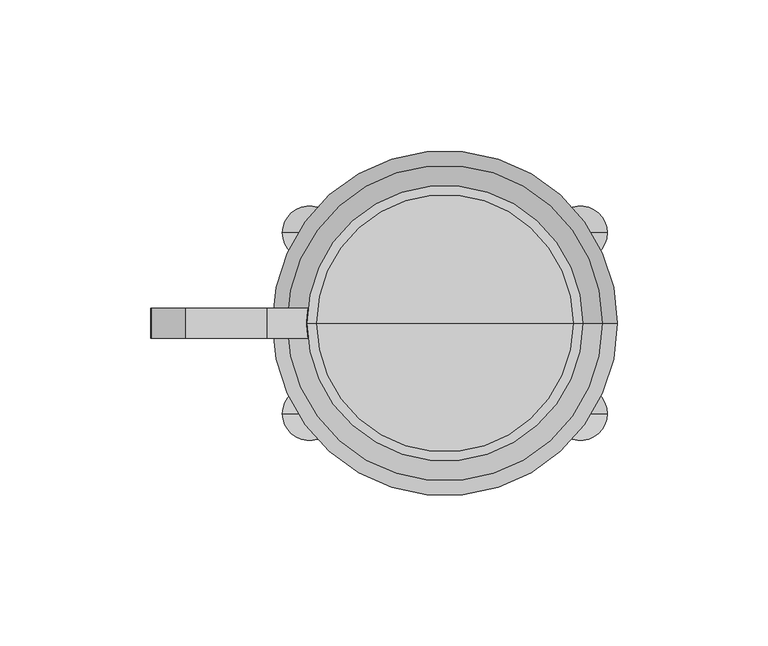
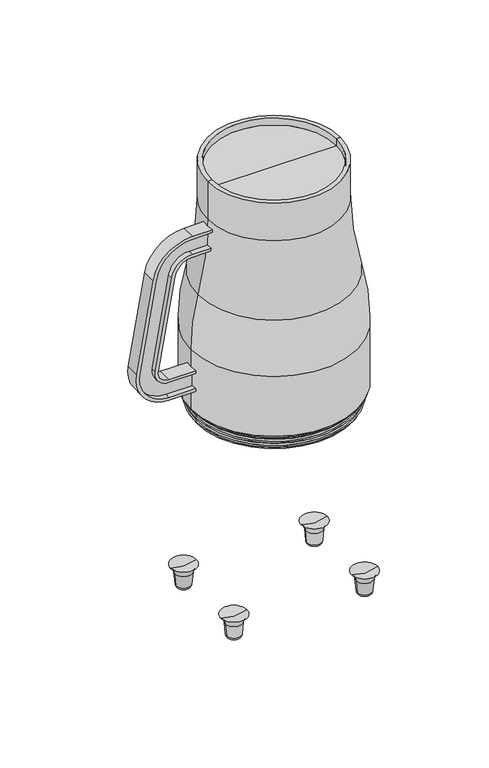
"""IFC4 building model written with IfcOpenShell, lengths in millimetres: proxy geometry, Smoothie_Maker_ : Smoothie_Maker_."""

from ifc_helpers import new_model, si_unit, point, frame, origin, place, context, project, spatial, polyline, circle_curve, ellipse_curve, trimmed, source, transform, mapped, element, save
from ifc_brep_helpers import plane_surface, cylinder_surface, revolved_surface, advanced_brep


def generic_models_ff15e8bf(model_context):
    return source(origin(), model_context, "Body", "AdvancedBrep", [
        advanced_brep(
        [(-43.932782, 5.0, 280.5), (-43.932782, -5.0, 280.5), (-43.932782, -5.0, 278.5), (-43.932782, -1.0, 278.5), (-43.932782, -1.0, 267.5), (-43.932782, -5.0, 267.5), (-43.932782, -5.0, 265.5), (-43.932782, 5.0, 265.5), (-43.932782, 5.0, 267.5), (-43.932782, 1.0, 267.5), (-43.932782, 1.0, 278.5), (-43.932782, 5.0, 278.5), (-58.932782, 5.0, 280.5), (-58.932782, -5.0, 280.5), (-86.0149953, -5.0, 257.7753249), (-97.361463, -5.0, 193.4263087), (-75.2032886, -5.0, 167.0192247), (-55.2032886, -5.0, 167.0192247), (-55.2032886, -5.0, 169.0192247), (-75.2032886, -5.0, 169.0192247), (-95.3918475, -5.0, 193.0790123), (-84.0453798, -5.0, 257.4280285), (-58.932782, -5.0, 278.5), (-58.932782, -1.0, 278.5), (-84.0453798, -1.0, 257.4280285), (-95.3918475, -1.0, 193.0790123), (-75.2032886, -1.0, 169.0192247), (-55.2032886, -1.0, 169.0192247), (-55.2032886, -1.0, 180.0192247), (-75.2032886, -1.0, 180.0192247), (-84.5589622, -1.0, 191.1688824), (-73.2124945, -1.0, 255.5178986), (-58.932782, -1.0, 267.5), (-58.932782, -5.0, 267.5), (-73.2124945, -5.0, 255.5178986), (-84.5589622, -5.0, 191.1688824), (-75.2032886, -5.0, 180.0192247), (-55.2032886, -5.0, 180.0192247), (-55.2032886, -5.0, 182.0192247), (-75.2032886, -5.0, 182.0192247), (-82.5893467, -5.0, 190.821586), (-71.242879, -5.0, 255.1706022), (-58.932782, -5.0, 265.5), (-58.932782, 5.0, 265.5), (-71.242879, 5.0, 255.1706022), (-82.5893467, 5.0, 190.821586), (-75.2032886, 5.0, 182.0192247), (-55.2032886, 5.0, 182.0192247), (-55.2032886, 5.0, 180.0192247), (-75.2032886, 5.0, 180.0192247), (-84.5589622, 5.0, 191.1688824), (-73.2124945, 5.0, 255.5178986), (-58.932782, 5.0, 267.5), (-58.932782, 1.0, 267.5), (-73.2124945, 1.0, 255.5178986), (-84.5589622, 1.0, 191.1688824), (-75.2032886, 1.0, 180.0192247), (-55.2032886, 1.0, 180.0192247), (-55.2032886, 1.0, 169.0192247), (-75.2032886, 1.0, 169.0192247), (-95.3918475, 1.0, 193.0790123), (-84.0453798, 1.0, 257.4280285), (-58.932782, 1.0, 278.5), (-58.932782, 5.0, 278.5), (-84.0453798, 5.0, 257.4280285), (-95.3918475, 5.0, 193.0790123), (-75.2032886, 5.0, 169.0192247), (-55.2032886, 5.0, 169.0192247), (-55.2032886, 5.0, 167.0192247), (-75.2032886, 5.0, 167.0192247), (-97.361463, 5.0, 193.4263087), (-86.0149953, 5.0, 257.7753249)],
        [
            (0, 1),
            (1, 2),
            (2, 3),
            (3, 4),
            (4, 5),
            (5, 6),
            (6, 7),
            (7, 8),
            (8, 9),
            (9, 10),
            (10, 11),
            (11, 0),
            (0, 12),
            (12, 13),
            (13, 1),
            (13, 14, circle_curve(frame((-58.932782, -5.0, 253.0), z_axis=(0.0, -1.0, 0.0), x_axis=(0.0, 0.0, 1.0)), 27.5)),
            (14, 15),
            (15, 16, circle_curve(frame((-75.2032886, -5.0, 189.5192247), z_axis=(0.0, -1.0, 0.0), x_axis=(-0.9848077530122076, 0.0, 0.17364817766693288)), 22.5)),
            (16, 17),
            (17, 18),
            (18, 19),
            (19, 20, circle_curve(frame((-75.2032886, -5.0, 189.5192247), z_axis=(0.0, 1.0, 0.0), x_axis=(-0.9848077530122076, 0.0, 0.17364817766693288)), 20.5)),
            (20, 21),
            (21, 22, circle_curve(frame((-58.932782, -5.0, 253.0), z_axis=(0.0, 1.0, 0.0), x_axis=(0.0, 0.0, 1.0)), 25.5)),
            (22, 2),
            (22, 23),
            (23, 3),
            (23, 24, circle_curve(frame((-58.932782, -1.0, 253.0), z_axis=(0.0, -1.0, 0.0), x_axis=(0.0, 0.0, 1.0)), 25.5)),
            (24, 25),
            (25, 26, circle_curve(frame((-75.2032886, -1.0, 189.5192247), z_axis=(0.0, -1.0, 0.0), x_axis=(-0.9848077530122076, 0.0, 0.17364817766693288)), 20.5)),
            (26, 27),
            (27, 28),
            (28, 29),
            (29, 30, circle_curve(frame((-75.2032886, -1.0, 189.5192247), z_axis=(0.0, 1.0, 0.0), x_axis=(-0.9848077530122076, 0.0, 0.17364817766693288)), 9.5)),
            (30, 31),
            (31, 32, circle_curve(frame((-58.932782, -1.0, 253.0), z_axis=(0.0, 1.0, 0.0), x_axis=(0.0, 0.0, 1.0)), 14.5)),
            (32, 4),
            (32, 33),
            (33, 5),
            (33, 34, circle_curve(frame((-58.932782, -5.0, 253.0), z_axis=(0.0, -1.0, 0.0), x_axis=(0.0, 0.0, 1.0)), 14.5)),
            (34, 35),
            (35, 36, circle_curve(frame((-75.2032886, -5.0, 189.5192247), z_axis=(0.0, -1.0, 0.0), x_axis=(-0.9848077530122076, 0.0, 0.17364817766693288)), 9.5)),
            (36, 37),
            (37, 38),
            (38, 39),
            (39, 40, circle_curve(frame((-75.2032886, -5.0, 189.5192247), z_axis=(0.0, 1.0, 0.0), x_axis=(-0.9848077530122076, 0.0, 0.17364817766693288)), 7.5)),
            (40, 41),
            (41, 42, circle_curve(frame((-58.932782, -5.0, 253.0), z_axis=(0.0, 1.0, 0.0), x_axis=(0.0, 0.0, 1.0)), 12.5)),
            (42, 6),
            (42, 43),
            (43, 7),
            (43, 44, circle_curve(frame((-58.932782, 5.0, 253.0), z_axis=(0.0, -1.0, 0.0), x_axis=(0.0, 0.0, 1.0)), 12.5)),
            (44, 45),
            (45, 46, circle_curve(frame((-75.2032886, 5.0, 189.5192247), z_axis=(0.0, -1.0, 0.0), x_axis=(-0.9848077530122076, 0.0, 0.17364817766693288)), 7.5)),
            (46, 47),
            (47, 48),
            (48, 49),
            (49, 50, circle_curve(frame((-75.2032886, 5.0, 189.5192247), z_axis=(0.0, 1.0, 0.0), x_axis=(-0.9848077530122076, 0.0, 0.17364817766693288)), 9.5)),
            (50, 51),
            (51, 52, circle_curve(frame((-58.932782, 5.0, 253.0), z_axis=(0.0, 1.0, 0.0), x_axis=(0.0, 0.0, 1.0)), 14.5)),
            (52, 8),
            (52, 53),
            (53, 9),
            (53, 54, circle_curve(frame((-58.932782, 1.0, 253.0), z_axis=(0.0, -1.0, 0.0), x_axis=(0.0, 0.0, 1.0)), 14.5)),
            (54, 55),
            (55, 56, circle_curve(frame((-75.2032886, 1.0, 189.5192247), z_axis=(0.0, -1.0, 0.0), x_axis=(-0.9848077530122076, 0.0, 0.17364817766693288)), 9.5)),
            (56, 57),
            (57, 58),
            (58, 59),
            (59, 60, circle_curve(frame((-75.2032886, 1.0, 189.5192247), z_axis=(0.0, 1.0, 0.0), x_axis=(-0.9848077530122076, 0.0, 0.17364817766693288)), 20.5)),
            (60, 61),
            (61, 62, circle_curve(frame((-58.932782, 1.0, 253.0), z_axis=(0.0, 1.0, 0.0), x_axis=(0.0, 0.0, 1.0)), 25.5)),
            (62, 10),
            (62, 63),
            (63, 11),
            (63, 64, circle_curve(frame((-58.932782, 5.0, 253.0), z_axis=(0.0, -1.0, 0.0), x_axis=(0.0, 0.0, 1.0)), 25.5)),
            (64, 65),
            (65, 66, circle_curve(frame((-75.2032886, 5.0, 189.5192247), z_axis=(0.0, -1.0, 0.0), x_axis=(-0.9848077530122076, 0.0, 0.17364817766693288)), 20.5)),
            (66, 67),
            (67, 68),
            (68, 69),
            (69, 70, circle_curve(frame((-75.2032886, 5.0, 189.5192247), z_axis=(0.0, 1.0, 0.0), x_axis=(-0.9848077530122076, 0.0, 0.17364817766693288)), 22.5)),
            (70, 71),
            (71, 12, circle_curve(frame((-58.932782, 5.0, 253.0), z_axis=(0.0, 1.0, 0.0), x_axis=(0.0, 0.0, 1.0)), 27.5)),
            (71, 14),
            (21, 24),
            (31, 34),
            (41, 44),
            (51, 54),
            (61, 64),
            (70, 15),
            (20, 25),
            (30, 35),
            (40, 45),
            (50, 55),
            (60, 65),
            (69, 16),
            (19, 26),
            (29, 36),
            (39, 46),
            (49, 56),
            (59, 66),
            (67, 58),
            (57, 48),
            (47, 38),
            (37, 28),
            (27, 18),
            (17, 68),
        ],
        [
            plane_surface(frame((-43.932782, 0.0, 273.0), z_axis=(1.0, 0.0, 0.0), x_axis=(0.0, -1.0, 0.0))),
            plane_surface(frame((-43.932782, 5.0, 280.5), z_axis=(0.0, 0.0, 1.0), x_axis=(-1.0, 0.0, 0.0))),
            plane_surface(frame((-43.932782, -5.0, 280.5), z_axis=(0.0, -1.0, 0.0), x_axis=(-1.0, 0.0, 0.0))),
            plane_surface(frame((-43.932782, -5.0, 278.5), z_axis=(0.0, 0.0, -1.0), x_axis=(-1.0, 0.0, 0.0))),
            plane_surface(frame((-43.932782, -1.0, 278.5), z_axis=(0.0, -1.0, 0.0), x_axis=(-1.0, 0.0, 0.0))),
            plane_surface(frame((-43.932782, -1.0, 267.5), z_axis=(0.0, 0.0, 1.0), x_axis=(-1.0, 0.0, 0.0))),
            plane_surface(frame((-43.932782, -5.0, 267.5), z_axis=(0.0, -1.0, 0.0), x_axis=(-1.0, 0.0, 0.0))),
            plane_surface(frame((-43.932782, -5.0, 265.5), z_axis=(0.0, 0.0, -1.0), x_axis=(-1.0, 0.0, 0.0))),
            plane_surface(frame((-43.932782, 5.0, 265.5), z_axis=(0.0, 1.0, 0.0), x_axis=(-1.0, 0.0, 0.0))),
            plane_surface(frame((-43.932782, 5.0, 267.5), z_axis=(0.0, 0.0, 1.0), x_axis=(-1.0, 0.0, 0.0))),
            plane_surface(frame((-43.932782, 1.0, 267.5), z_axis=(0.0, 1.0, 0.0), x_axis=(-1.0, 0.0, 0.0))),
            plane_surface(frame((-43.932782, 1.0, 278.5), z_axis=(0.0, 0.0, -1.0), x_axis=(-1.0, 0.0, 0.0))),
            plane_surface(frame((-43.932782, 5.0, 278.5), z_axis=(0.0, 1.0, 0.0), x_axis=(-1.0, 0.0, 0.0))),
            cylinder_surface(frame((-58.932782, 0.0, 253.0), z_axis=(0.0, -1.0, 0.0), x_axis=(0.0, 0.0, 1.0)), 27.5),
            revolved_surface(polyline([(-58.932782, -5.0, 278.5), (-58.932782, -1.0, 278.5)]), (-58.932782, 0.0, 253.0), (0.0, -1.0, 0.0)),
            cylinder_surface(frame((-58.932782, 0.0, 253.0), z_axis=(0.0, -1.0, 0.0), x_axis=(0.0, 0.0, 1.0)), 14.5),
            revolved_surface(polyline([(-58.932782, -5.0, 265.5), (-58.932782, 5.0, 265.5)]), (-58.932782, 0.0, 253.0), (0.0, -1.0, 0.0)),
            revolved_surface(polyline([(-58.932782, 1.0, 278.5), (-58.932782, 5.0, 278.5)]), (-58.932782, 0.0, 253.0), (0.0, -1.0, 0.0)),
            plane_surface(frame((-86.0149953, 5.0, 257.7753249), z_axis=(-0.9848077530122079, 0.0, 0.1736481776669317), x_axis=(-0.1736481776669317, 0.0, -0.9848077530122079))),
            plane_surface(frame((-84.0453798, -5.0, 257.4280285), z_axis=(0.9848077530122078, 0.0, -0.1736481776669319), x_axis=(-0.1736481776669319, 0.0, -0.9848077530122078))),
            plane_surface(frame((-73.2124945, -1.0, 255.5178986), z_axis=(-0.9848077530122078, 0.0, 0.17364817766693202), x_axis=(-0.17364817766693202, 0.0, -0.9848077530122078))),
            plane_surface(frame((-71.242879, -5.0, 255.1706022), z_axis=(0.9848077530122078, 0.0, -0.1736481776669318), x_axis=(-0.1736481776669318, 0.0, -0.9848077530122078))),
            plane_surface(frame((-73.2124945, 5.0, 255.5178986), z_axis=(-0.9848077530122078, 0.0, 0.17364817766693202), x_axis=(-0.17364817766693202, 0.0, -0.9848077530122078))),
            plane_surface(frame((-84.0453798, 1.0, 257.4280285), z_axis=(0.9848077530122078, 0.0, -0.1736481776669319), x_axis=(-0.1736481776669319, 0.0, -0.9848077530122078))),
            cylinder_surface(frame((-75.2032886, 0.0, 189.5192247), z_axis=(0.0, -1.0, 0.0), x_axis=(-0.9848077530122076, 0.0, 0.17364817766693288)), 22.5),
            revolved_surface(polyline([(-95.39184753675025, -5.0, 193.07901234217212), (-95.39184753675025, -1.0, 193.07901234217212)]), (-75.2032886, 0.0, 189.5192247), (0.0, -1.0, 0.0)),
            cylinder_surface(frame((-75.2032886, 0.0, 189.5192247), z_axis=(0.0, -1.0, 0.0), x_axis=(-0.9848077530122076, 0.0, 0.17364817766693288)), 9.5),
            revolved_surface(polyline([(-82.58934674759155, -5.0, 190.82158603250198), (-82.58934674759155, 5.0, 190.82158603250198)]), (-75.2032886, 0.0, 189.5192247), (0.0, -1.0, 0.0)),
            revolved_surface(polyline([(-95.39184753675025, 1.0, 193.07901234217212), (-95.39184753675025, 5.0, 193.07901234217212)]), (-75.2032886, 0.0, 189.5192247), (0.0, -1.0, 0.0)),
            plane_surface(frame((-55.2032886, 0.0, 174.5192247), z_axis=(1.0, 0.0, 0.0), x_axis=(0.0, -1.0, 0.0))),
            plane_surface(frame((-75.2032886, 5.0, 167.0192247), z_axis=(0.0, 0.0, -1.0), x_axis=(1.0, 0.0, 0.0))),
            plane_surface(frame((-75.2032886, -5.0, 169.0192247), z_axis=(0.0, 0.0, 1.0), x_axis=(1.0, 0.0, 0.0))),
            plane_surface(frame((-75.2032886, -1.0, 180.0192247), z_axis=(0.0, 0.0, -1.0), x_axis=(1.0, 0.0, 0.0))),
            plane_surface(frame((-75.2032886, -5.0, 182.0192247), z_axis=(0.0, 0.0, 1.0), x_axis=(1.0, 0.0, 0.0))),
            plane_surface(frame((-75.2032886, 5.0, 180.0192247), z_axis=(0.0, 0.0, -1.0), x_axis=(1.0, 0.0, 0.0))),
            plane_surface(frame((-75.2032886, 1.0, 169.0192247), z_axis=(0.0, 0.0, 1.0), x_axis=(1.0, 0.0, 0.0))),
        ],
        [
            (0, [[1, 2, 3, 4, 5, 6, 7, 8, 9, 10, 11, 12]]),
            (1, [[-1, 13, 14, 15]]),
            (2, [[-2, -15, 16, 17, 18, 19, 20, 21, 22, 23, 24, 25]]),
            (3, [[-3, -25, 26, 27]]),
            (4, [[-4, -27, 28, 29, 30, 31, 32, 33, 34, 35, 36, 37]]),
            (5, [[-5, -37, 38, 39]]),
            (6, [[-6, -39, 40, 41, 42, 43, 44, 45, 46, 47, 48, 49]]),
            (7, [[-7, -49, 50, 51]]),
            (8, [[-8, -51, 52, 53, 54, 55, 56, 57, 58, 59, 60, 61]]),
            (9, [[-9, -61, 62, 63]]),
            (10, [[-10, -63, 64, 65, 66, 67, 68, 69, 70, 71, 72, 73]]),
            (11, [[-11, -73, 74, 75]]),
            (12, [[-12, -75, 76, 77, 78, 79, 80, 81, 82, 83, 84, -13]]),
            (13, [[-16, -14, -84, 85]]),
            (14, [[-28, -26, -24, 86]]),
            (15, [[-40, -38, -36, 87]]),
            (16, [[-52, -50, -48, 88]]),
            (15, [[-64, -62, -60, 89]]),
            (17, [[-76, -74, -72, 90]]),
            (18, [[-85, -83, 91, -17]]),
            (19, [[-86, -23, 92, -29]]),
            (20, [[-87, -35, 93, -41]]),
            (21, [[-88, -47, 94, -53]]),
            (22, [[-89, -59, 95, -65]]),
            (23, [[-90, -71, 96, -77]]),
            (24, [[-18, -91, -82, 97]]),
            (25, [[-30, -92, -22, 98]]),
            (26, [[-42, -93, -34, 99]]),
            (27, [[-54, -94, -46, 100]]),
            (26, [[-66, -95, -58, 101]]),
            (28, [[-78, -96, -70, 102]]),
            (29, [[-80, 103, -68, 104, -56, 105, -44, 106, -32, 107, -20, 108]]),
            (30, [[-97, -81, -108, -19]]),
            (31, [[-98, -21, -107, -31]]),
            (32, [[-99, -33, -106, -43]]),
            (33, [[-100, -45, -105, -55]]),
            (34, [[-101, -57, -104, -67]]),
            (35, [[-102, -69, -103, -79]]),
        ],
    ),
        advanced_brep(
        [(53.5777998, 0.0, 146.8454413), (-53.5777998, 0.0, 146.8454413), (-54.2311845, 0.0, 147.4988261), (54.2311845, 0.0, 147.4988261), (53.5777998, 0.0, 145.1522109), (-53.5777998, 0.0, 145.1522109), (54.2311845, 0.0, 144.4988261), (-54.2311845, 0.0, 144.4988261), (53.5777998, 0.0, 143.8454413), (-53.5777998, 0.0, 143.8454413), (53.5777998, 0.0, 142.1522109), (-53.5777998, 0.0, 142.1522109), (54.2311845, 0.0, 141.4988261), (-54.2311845, 0.0, 141.4988261), (53.5777998, 0.0, 140.8454413), (-53.5777998, 0.0, 140.8454413), (53.5777998, 0.0, 140.0), (-53.5777998, 0.0, 140.0), (51.2888999, 0.0, 140.0), (-51.2888999, 0.0, 140.0), (51.2888999, 0.0, 195.0), (-51.2888999, 0.0, 195.0), (46.661713, 0.0, 231.2107577), (-46.661713, 0.0, 231.2107577), (0.0, 0.0, 302.0), (-39.7147747, 0.0, 302.0), (39.7147747, 0.0, 302.0), (42.7147747, 0.0, 308.0), (-42.7147747, 0.0, 308.0), (0.0, 0.0, 308.0), (42.7147747, 0.0, 313.0), (-42.7147747, 0.0, 313.0), (45.7147747, 0.0, 313.0), (-45.7147747, 0.0, 313.0), (45.7147747, 0.0, 285.575084), (-45.7147747, 0.0, 285.575084), (57.2888999, 0.0, 195.0), (-57.2888999, 0.0, 195.0), (-52.4689135, 0.0, 232.7195393), (52.4689135, 0.0, 232.7195393), (57.2888999, 0.0, 151.4890625), (-57.2888999, 0.0, 151.4890625), (55.7998373, 0.0, 150.0), (-55.7998373, 0.0, 150.0), (53.5777998, 0.0, 150.0), (-53.5777998, 0.0, 150.0), (53.5777998, 0.0, 148.1522109), (-53.5777998, 0.0, 148.1522109), (39.7147747, 0.0, 285.575084), (-39.7147747, 0.0, 285.575084)],
        [
            (0, 1, circle_curve(frame((0.0, 0.0, 146.8454413), z_axis=(0.0, 0.0, 1.0), x_axis=(-1.0, 0.0, 0.0)), 53.5777998)),
            (1, 2),
            (2, 3, circle_curve(frame((0.0, 0.0, 147.4988261), z_axis=(0.0, 0.0, -1.0), x_axis=(-1.0, 0.0, 0.0)), 54.2311845)),
            (3, 0),
            (1, 0, circle_curve(frame((0.0, 0.0, 146.8454413), z_axis=(0.0, 0.0, 1.0), x_axis=(-1.0, 0.0, 0.0)), 53.5777998)),
            (3, 2, circle_curve(frame((0.0, 0.0, 147.4988261), z_axis=(0.0, 0.0, -1.0), x_axis=(-1.0, 0.0, 0.0)), 54.2311845)),
            (4, 5, circle_curve(frame((0.0, 0.0, 145.1522109), z_axis=(0.0, 0.0, 1.0), x_axis=(-1.0, 0.0, 0.0)), 53.5777998)),
            (5, 1),
            (0, 4),
            (5, 4, circle_curve(frame((0.0, 0.0, 145.1522109), z_axis=(0.0, 0.0, 1.0), x_axis=(-1.0, 0.0, 0.0)), 53.5777998)),
            (6, 7, circle_curve(frame((0.0, 0.0, 144.4988261), z_axis=(0.0, 0.0, 1.0), x_axis=(-1.0, 0.0, 0.0)), 54.2311845)),
            (7, 5),
            (4, 6),
            (7, 6, circle_curve(frame((0.0, 0.0, 144.4988261), z_axis=(0.0, 0.0, 1.0), x_axis=(-1.0, 0.0, 0.0)), 54.2311845)),
            (8, 9, circle_curve(frame((0.0, 0.0, 143.8454413), z_axis=(0.0, 0.0, 1.0), x_axis=(-1.0, 0.0, 0.0)), 53.5777998)),
            (9, 7),
            (6, 8),
            (9, 8, circle_curve(frame((0.0, 0.0, 143.8454413), z_axis=(0.0, 0.0, 1.0), x_axis=(-1.0, 0.0, 0.0)), 53.5777998)),
            (10, 11, circle_curve(frame((0.0, 0.0, 142.1522109), z_axis=(0.0, 0.0, 1.0), x_axis=(-1.0, 0.0, 0.0)), 53.5777998)),
            (11, 9),
            (8, 10),
            (11, 10, circle_curve(frame((0.0, 0.0, 142.1522109), z_axis=(0.0, 0.0, 1.0), x_axis=(-1.0, 0.0, 0.0)), 53.5777998)),
            (12, 13, circle_curve(frame((0.0, 0.0, 141.4988261), z_axis=(0.0, 0.0, 1.0), x_axis=(-1.0, 0.0, 0.0)), 54.2311845)),
            (13, 11),
            (10, 12),
            (13, 12, circle_curve(frame((0.0, 0.0, 141.4988261), z_axis=(0.0, 0.0, 1.0), x_axis=(-1.0, 0.0, 0.0)), 54.2311845)),
            (14, 15, circle_curve(frame((0.0, 0.0, 140.8454413), z_axis=(0.0, 0.0, 1.0), x_axis=(-1.0, 0.0, 0.0)), 53.5777998)),
            (15, 13),
            (12, 14),
            (15, 14, circle_curve(frame((0.0, 0.0, 140.8454413), z_axis=(0.0, 0.0, 1.0), x_axis=(-1.0, 0.0, 0.0)), 53.5777998)),
            (16, 17, circle_curve(frame((0.0, 0.0, 140.0), z_axis=(0.0, 0.0, 1.0), x_axis=(-1.0, 0.0, 0.0)), 53.5777998)),
            (17, 15),
            (14, 16),
            (17, 16, circle_curve(frame((0.0, 0.0, 140.0), z_axis=(0.0, 0.0, 1.0), x_axis=(-1.0, 0.0, 0.0)), 53.5777998)),
            (18, 19, circle_curve(frame((0.0, 0.0, 140.0), z_axis=(0.0, 0.0, 1.0), x_axis=(-1.0, 0.0, 0.0)), 51.2888999)),
            (19, 17),
            (16, 18),
            (19, 18, circle_curve(frame((0.0, 0.0, 140.0), z_axis=(0.0, 0.0, 1.0), x_axis=(-1.0, 0.0, 0.0)), 51.2888999)),
            (20, 21, circle_curve(frame((0.0, 0.0, 195.0), z_axis=(0.0, 0.0, 1.0), x_axis=(-1.0, 0.0, 0.0)), 51.2888999)),
            (21, 19),
            (18, 20),
            (21, 20, circle_curve(frame((0.0, 0.0, 195.0), z_axis=(0.0, 0.0, 1.0), x_axis=(-1.0, 0.0, 0.0)), 51.2888999)),
            (22, 23, circle_curve(frame((0.0, 0.0, 231.2107577), z_axis=(0.0, 0.0, 1.0), x_axis=(-1.0, 0.0, 0.0)), 46.661713)),
            (23, 21, circle_curve(frame((92.7111001, 0.0, 195.0), z_axis=(0.0, -1.0, 0.0), x_axis=(1.0, 0.0, 0.0)), 144.0)),
            (20, 22, circle_curve(frame((-92.7111001, 0.0, 195.0), z_axis=(0.0, -1.0, 0.0), x_axis=(-1.0, 0.0, 0.0)), 144.0)),
            (23, 22, circle_curve(frame((0.0, 0.0, 231.2107577), z_axis=(0.0, 0.0, 1.0), x_axis=(-1.0, 0.0, 0.0)), 46.661713)),
            (24, 25),
            (25, 26, circle_curve(frame((0.0, 0.0, 302.0), z_axis=(0.0, 0.0, -1.0), x_axis=(-1.0, 0.0, 0.0)), 39.7147747)),
            (26, 24),
            (26, 25, circle_curve(frame((0.0, 0.0, 302.0), z_axis=(0.0, 0.0, -1.0), x_axis=(-1.0, 0.0, 0.0)), 39.7147747)),
            (27, 28, circle_curve(frame((0.0, 0.0, 308.0), z_axis=(0.0, 0.0, 1.0), x_axis=(-1.0, 0.0, 0.0)), 42.7147747)),
            (28, 29),
            (29, 27),
            (28, 27, circle_curve(frame((0.0, 0.0, 308.0), z_axis=(0.0, 0.0, 1.0), x_axis=(-1.0, 0.0, 0.0)), 42.7147747)),
            (30, 31, circle_curve(frame((0.0, 0.0, 313.0), z_axis=(0.0, 0.0, 1.0), x_axis=(-1.0, 0.0, 0.0)), 42.7147747)),
            (31, 28),
            (27, 30),
            (31, 30, circle_curve(frame((0.0, 0.0, 313.0), z_axis=(0.0, 0.0, 1.0), x_axis=(-1.0, 0.0, 0.0)), 42.7147747)),
            (32, 33, circle_curve(frame((0.0, 0.0, 313.0), z_axis=(0.0, 0.0, 1.0), x_axis=(-1.0, 0.0, 0.0)), 45.7147747)),
            (33, 31),
            (30, 32),
            (33, 32, circle_curve(frame((0.0, 0.0, 313.0), z_axis=(0.0, 0.0, 1.0), x_axis=(-1.0, 0.0, 0.0)), 45.7147747)),
            (34, 35, circle_curve(frame((0.0, 0.0, 285.575084), z_axis=(0.0, 0.0, 1.0), x_axis=(-1.0, 0.0, 0.0)), 45.7147747)),
            (35, 33),
            (32, 34),
            (35, 34, circle_curve(frame((0.0, 0.0, 285.575084), z_axis=(0.0, 0.0, 1.0), x_axis=(-1.0, 0.0, 0.0)), 45.7147747)),
            (36, 37, circle_curve(frame((0.0, 0.0, 195.0), z_axis=(0.0, 0.0, 1.0), x_axis=(-1.0, 0.0, 0.0)), 57.2888999)),
            (37, 38, circle_curve(frame((92.7111001, 0.0, 195.0), z_axis=(0.0, 1.0, 0.0), x_axis=(1.0, 0.0, 0.0)), 150.0)),
            (38, 39, circle_curve(frame((0.0, 0.0, 232.7195393), z_axis=(0.0, 0.0, -1.0), x_axis=(-1.0, 0.0, 0.0)), 52.4689135)),
            (39, 36, circle_curve(frame((-92.7111001, 0.0, 195.0), z_axis=(0.0, 1.0, 0.0), x_axis=(-1.0, 0.0, 0.0)), 150.0)),
            (37, 36, circle_curve(frame((0.0, 0.0, 195.0), z_axis=(0.0, 0.0, 1.0), x_axis=(-1.0, 0.0, 0.0)), 57.2888999)),
            (39, 38, circle_curve(frame((0.0, 0.0, 232.7195393), z_axis=(0.0, 0.0, -1.0), x_axis=(-1.0, 0.0, 0.0)), 52.4689135)),
            (40, 41, circle_curve(frame((0.0, 0.0, 151.4890625), z_axis=(0.0, 0.0, 1.0), x_axis=(-1.0, 0.0, 0.0)), 57.2888999)),
            (41, 37),
            (36, 40),
            (41, 40, circle_curve(frame((0.0, 0.0, 151.4890625), z_axis=(0.0, 0.0, 1.0), x_axis=(-1.0, 0.0, 0.0)), 57.2888999)),
            (42, 43, circle_curve(frame((0.0, 0.0, 150.0), z_axis=(0.0, 0.0, 1.0), x_axis=(-1.0, 0.0, 0.0)), 55.7998373)),
            (43, 41, circle_curve(frame((-55.7998373, 0.0, 151.4890625), z_axis=(0.0, 1.0, 0.0), x_axis=(1.0, 0.0, 0.0)), 1.4890625)),
            (40, 42, circle_curve(frame((55.7998373, 0.0, 151.4890625), z_axis=(0.0, 1.0, 0.0), x_axis=(-1.0, 0.0, 0.0)), 1.4890625)),
            (43, 42, circle_curve(frame((0.0, 0.0, 150.0), z_axis=(0.0, 0.0, 1.0), x_axis=(-1.0, 0.0, 0.0)), 55.7998373)),
            (44, 45, circle_curve(frame((0.0, 0.0, 150.0), z_axis=(0.0, 0.0, 1.0), x_axis=(-1.0, 0.0, 0.0)), 53.5777998)),
            (45, 43),
            (42, 44),
            (45, 44, circle_curve(frame((0.0, 0.0, 150.0), z_axis=(0.0, 0.0, 1.0), x_axis=(-1.0, 0.0, 0.0)), 53.5777998)),
            (46, 47, circle_curve(frame((0.0, 0.0, 148.1522109), z_axis=(0.0, 0.0, 1.0), x_axis=(-1.0, 0.0, 0.0)), 53.5777998)),
            (47, 45),
            (44, 46),
            (47, 46, circle_curve(frame((0.0, 0.0, 148.1522109), z_axis=(0.0, 0.0, 1.0), x_axis=(-1.0, 0.0, 0.0)), 53.5777998)),
            (2, 47),
            (46, 3),
            (48, 49, circle_curve(frame((0.0, 0.0, 285.575084), z_axis=(0.0, 0.0, 1.0), x_axis=(-1.0, 0.0, 0.0)), 39.7147747)),
            (49, 23, circle_curve(frame((-255.9064119, 0.0, 285.575084), z_axis=(0.0, 1.0, 0.0), x_axis=(1.0, 0.0, 0.0)), 216.1916373)),
            (22, 48, circle_curve(frame((255.9064119, 0.0, 285.575084), z_axis=(0.0, 1.0, 0.0), x_axis=(-1.0, 0.0, 0.0)), 216.1916373)),
            (49, 48, circle_curve(frame((0.0, 0.0, 285.575084), z_axis=(0.0, 0.0, 1.0), x_axis=(-1.0, 0.0, 0.0)), 39.7147747)),
            (25, 49),
            (48, 26),
            (38, 35, circle_curve(frame((-255.9064119, 0.0, 285.575084), z_axis=(0.0, -1.0, 0.0), x_axis=(1.0, 0.0, 0.0)), 210.1916373)),
            (34, 39, circle_curve(frame((255.9064119, 0.0, 285.575084), z_axis=(0.0, -1.0, 0.0), x_axis=(-1.0, 0.0, 0.0)), 210.1916373)),
        ],
        [
            revolved_surface(polyline([(-54.2311845, 0.0, 147.4988261), (-53.5777998, 0.0, 146.8454413)]), (0.0, 0.0, 308.0), (0.0, 0.0, -1.0)),
            cylinder_surface(frame((0.0, 0.0, 308.0), z_axis=(0.0, 0.0, -1.0), x_axis=(-1.0, 0.0, 0.0)), 53.5777998),
            revolved_surface(polyline([(-53.5777998, 0.0, 145.1522109), (-54.2311845, 0.0, 144.4988261)]), (0.0, 0.0, 308.0), (0.0, 0.0, -1.0)),
            revolved_surface(polyline([(-54.2311845, 0.0, 144.4988261), (-53.5777998, 0.0, 143.8454413)]), (0.0, 0.0, 308.0), (0.0, 0.0, -1.0)),
            revolved_surface(polyline([(-53.5777998, 0.0, 142.1522109), (-54.2311845, 0.0, 141.4988261)]), (0.0, 0.0, 308.0), (0.0, 0.0, -1.0)),
            revolved_surface(polyline([(-54.2311845, 0.0, 141.4988261), (-53.5777998, 0.0, 140.8454413)]), (0.0, 0.0, 308.0), (0.0, 0.0, -1.0)),
            plane_surface(frame((0.0, 0.0, 140.0), z_axis=(0.0, 0.0, -1.0), x_axis=(-1.0, 0.0, 0.0))),
            revolved_surface(polyline([(-51.2888999, 0.0, 140.0), (-51.2888999, 0.0, 195.0)]), (0.0, 0.0, 308.0), (0.0, 0.0, -1.0)),
            revolved_surface(trimmed(ellipse_curve(frame((92.7111001, 0.0, 195.0), z_axis=(0.0, 1.0, 0.0), x_axis=(1.0, 0.0, 0.0)), 144.0, 144.0), [point((-51.2888999, 0.0, 195.0))], [point((-46.661713, 0.0, 231.2107577))], True, "CARTESIAN"), (0.0, 0.0, 308.0), (0.0, 0.0, -1.0)),
            plane_surface(frame((0.0, 0.0, 302.0), z_axis=(0.0, 0.0, -1.0), x_axis=(-1.0, 0.0, 0.0))),
            plane_surface(frame((0.0, 0.0, 308.0), z_axis=(0.0, 0.0, 1.0), x_axis=(-1.0, 0.0, 0.0))),
            revolved_surface(polyline([(-42.7147747, 0.0, 308.0), (-42.7147747, 0.0, 313.0)]), (0.0, 0.0, 308.0), (0.0, 0.0, -1.0)),
            plane_surface(frame((0.0, 0.0, 313.0), z_axis=(0.0, 0.0, 1.0), x_axis=(-1.0, 0.0, 0.0))),
            cylinder_surface(frame((0.0, 0.0, 308.0), z_axis=(0.0, 0.0, -1.0), x_axis=(-1.0, 0.0, 0.0)), 45.7147747),
            revolved_surface(trimmed(ellipse_curve(frame((92.7111001, 0.0, 195.0), z_axis=(0.0, -1.0, 0.0), x_axis=(1.0, 0.0, 0.0)), 150.0, 150.0), [point((-52.4689135, 0.0, 232.7195393))], [point((-57.2888999, 0.0, 195.0))], True, "CARTESIAN"), (0.0, 0.0, 308.0), (0.0, 0.0, -1.0)),
            cylinder_surface(frame((0.0, 0.0, 308.0), z_axis=(0.0, 0.0, -1.0), x_axis=(-1.0, 0.0, 0.0)), 57.2888999),
            revolved_surface(trimmed(ellipse_curve(frame((-55.7998373, 0.0, 151.4890625), z_axis=(0.0, -1.0, 0.0), x_axis=(1.0, 0.0, 0.0)), 1.4890625, 1.4890625), [point((-57.2888999, 0.0, 151.4890625))], [point((-55.7998373, 0.0, 150.0))], True, "CARTESIAN"), (0.0, 0.0, 308.0), (0.0, 0.0, -1.0)),
            plane_surface(frame((0.0, 0.0, 150.0), z_axis=(0.0, 0.0, -1.0), x_axis=(-1.0, 0.0, 0.0))),
            revolved_surface(polyline([(-53.5777998, 0.0, 148.1522109), (-54.2311845, 0.0, 147.4988261)]), (0.0, 0.0, 308.0), (0.0, 0.0, -1.0)),
            revolved_surface(trimmed(ellipse_curve(frame((-255.9064119, 0.0, 285.575084), z_axis=(0.0, -1.0, 0.0), x_axis=(1.0, 0.0, 0.0)), 216.1916373, 216.1916373), [point((-46.661713, 0.0, 231.2107577))], [point((-39.7147747, 0.0, 285.575084))], True, "CARTESIAN"), (0.0, 0.0, 308.0), (0.0, 0.0, -1.0)),
            revolved_surface(polyline([(-39.7147747, 0.0, 285.575084), (-39.7147747, 0.0, 302.0)]), (0.0, 0.0, 308.0), (0.0, 0.0, -1.0)),
            revolved_surface(trimmed(ellipse_curve(frame((-255.9064119, 0.0, 285.575084), z_axis=(0.0, 1.0, 0.0), x_axis=(1.0, 0.0, 0.0)), 210.1916373, 210.1916373), [point((-45.7147747, 0.0, 285.575084))], [point((-52.4689135, 0.0, 232.7195393))], True, "CARTESIAN"), (0.0, 0.0, 308.0), (0.0, 0.0, -1.0)),
        ],
        [
            (0, [[1, 2, 3, 4]]),
            (0, [[5, -4, 6, -2]]),
            (1, [[7, 8, -1, 9]]),
            (1, [[10, -9, -5, -8]]),
            (2, [[11, 12, -7, 13]]),
            (2, [[14, -13, -10, -12]]),
            (3, [[15, 16, -11, 17]]),
            (3, [[18, -17, -14, -16]]),
            (1, [[19, 20, -15, 21]]),
            (1, [[22, -21, -18, -20]]),
            (4, [[23, 24, -19, 25]]),
            (4, [[26, -25, -22, -24]]),
            (5, [[27, 28, -23, 29]]),
            (5, [[30, -29, -26, -28]]),
            (1, [[31, 32, -27, 33]]),
            (1, [[34, -33, -30, -32]]),
            (6, [[35, 36, -31, 37]]),
            (6, [[38, -37, -34, -36]]),
            (7, [[39, 40, -35, 41]]),
            (7, [[42, -41, -38, -40]]),
            (8, [[43, 44, -39, 45]]),
            (8, [[46, -45, -42, -44]]),
            (9, [[47, 48, 49]]),
            (9, [[-49, 50, -47]]),
            (10, [[51, 52, 53]]),
            (10, [[54, -53, -52]]),
            (11, [[55, 56, -51, 57]]),
            (11, [[58, -57, -54, -56]]),
            (12, [[59, 60, -55, 61]]),
            (12, [[62, -61, -58, -60]]),
            (13, [[63, 64, -59, 65]]),
            (13, [[66, -65, -62, -64]]),
            (14, [[67, 68, 69, 70]]),
            (14, [[71, -70, 72, -68]]),
            (15, [[73, 74, -67, 75]]),
            (15, [[76, -75, -71, -74]]),
            (16, [[77, 78, -73, 79]]),
            (16, [[80, -79, -76, -78]]),
            (17, [[81, 82, -77, 83]]),
            (17, [[84, -83, -80, -82]]),
            (1, [[85, 86, -81, 87]]),
            (1, [[88, -87, -84, -86]]),
            (18, [[-3, 89, -85, 90]]),
            (18, [[-6, -90, -88, -89]]),
            (19, [[91, 92, -43, 93]]),
            (19, [[94, -93, -46, -92]]),
            (20, [[-48, 95, -91, 96]]),
            (20, [[-50, -96, -94, -95]]),
            (21, [[-69, 97, -63, 98]]),
            (21, [[-72, -98, -66, -97]]),
        ],
    ),
        advanced_brep(
        [(40.0092654, 30.0, 1.9592283), (49.9712124, 30.0, 1.9592283), (50.7396487, 30.0, 10.7424955), (39.2408291, 30.0, 10.7424955), (41.9684938, 30.0, 0.0), (48.0119841, 30.0, 0.0), (44.9902389, 30.0, 0.0), (36.0562353, 30.0, 16.2583737), (53.9242425, 30.0, 16.2583737), (44.9902389, 30.0, 14.456439)],
        [
            (0, 1, circle_curve(frame((44.9902389, 30.0, 1.9592283), z_axis=(0.0, 0.0, 1.0), x_axis=(1.0, 0.0, 0.0)), 4.9809735)),
            (1, 2),
            (2, 3, circle_curve(frame((44.9902389, 30.0, 10.7424955), z_axis=(0.0, 0.0, -1.0), x_axis=(1.0, 0.0, 0.0)), 5.7494098)),
            (3, 0),
            (1, 0, circle_curve(frame((44.9902389, 30.0, 1.9592283), z_axis=(0.0, 0.0, 1.0), x_axis=(1.0, 0.0, 0.0)), 4.9809735)),
            (3, 2, circle_curve(frame((44.9902389, 30.0, 10.7424955), z_axis=(0.0, 0.0, -1.0), x_axis=(1.0, 0.0, 0.0)), 5.7494098)),
            (4, 5, circle_curve(frame((44.9902389, 30.0, 0.0), z_axis=(0.0, 0.0, 1.0), x_axis=(1.0, 0.0, 0.0)), 3.0217452)),
            (5, 1, circle_curve(frame((48.0119841, 30.0, 1.9592283), z_axis=(0.0, -1.0, 0.0), x_axis=(-1.0, 0.0, 0.0)), 1.9592283)),
            (0, 4, circle_curve(frame((41.9684938, 30.0, 1.9592283), z_axis=(0.0, -1.0, 0.0), x_axis=(1.0, 0.0, 0.0)), 1.9592283)),
            (5, 4, circle_curve(frame((44.9902389, 30.0, 0.0), z_axis=(0.0, 0.0, 1.0), x_axis=(1.0, 0.0, 0.0)), 3.0217452)),
            (6, 5),
            (4, 6),
            (7, 8, circle_curve(frame((44.9902389, 30.0, 16.2583737), z_axis=(0.0, 0.0, 1.0), x_axis=(1.0, 0.0, 0.0)), 8.9340036)),
            (8, 9, circle_curve(frame((39.739977, 30.0, 63.535659), z_axis=(0.0, 1.0, 0.0), x_axis=(-1.0, 0.0, 0.0)), 49.3592453)),
            (9, 7, circle_curve(frame((50.2405009, 30.0, 63.535659), z_axis=(0.0, 1.0, 0.0), x_axis=(1.0, 0.0, 0.0)), 49.3592453)),
            (8, 7, circle_curve(frame((44.9902389, 30.0, 16.2583737), z_axis=(0.0, 0.0, 1.0), x_axis=(1.0, 0.0, 0.0)), 8.9340036)),
            (2, 8, circle_curve(frame((58.2463651, 30.0, 10.0857429), z_axis=(0.0, 1.0, 0.0), x_axis=(-1.0, 0.0, 0.0)), 7.5353909)),
            (7, 3, circle_curve(frame((31.7341127, 30.0, 10.0857429), z_axis=(0.0, 1.0, 0.0), x_axis=(1.0, 0.0, 0.0)), 7.5353909)),
        ],
        [
            revolved_surface(polyline([(50.7396487, 30.0, 10.7424955), (49.9712124, 30.0, 1.9592283)]), (44.9902389, 30.0, 13.518939), (0.0, 0.0, -1.0)),
            revolved_surface(trimmed(ellipse_curve(frame((48.0119841, 30.0, 1.9592283), z_axis=(0.0, 1.0, 0.0), x_axis=(-1.0, 0.0, 0.0)), 1.9592283, 1.9592283), [point((49.9712124, 30.0, 1.9592283))], [point((48.0119841, 30.0, 0.0))], True, "CARTESIAN"), (44.9902389, 30.0, 13.518939), (0.0, 0.0, -1.0)),
            plane_surface(frame((44.9902389, 30.0, 0.0), z_axis=(0.0, 0.0, -1.0), x_axis=(1.0, 0.0, 0.0))),
            revolved_surface(trimmed(ellipse_curve(frame((39.739977, 30.0, 63.535659), z_axis=(0.0, -1.0, 0.0), x_axis=(-1.0, 0.0, 0.0)), 49.3592453, 49.3592453), [point((44.9902389, 30.0, 14.456439))], [point((53.9242425, 30.0, 16.2583737))], True, "CARTESIAN"), (44.9902389, 30.0, 13.518939), (0.0, 0.0, -1.0)),
            revolved_surface(trimmed(ellipse_curve(frame((58.2463651, 30.0, 10.0857429), z_axis=(0.0, -1.0, 0.0), x_axis=(-1.0, 0.0, 0.0)), 7.5353909, 7.5353909), [point((53.9242425, 30.0, 16.2583737))], [point((50.7396487, 30.0, 10.7424955))], True, "CARTESIAN"), (44.9902389, 30.0, 13.518939), (0.0, 0.0, -1.0)),
        ],
        [
            (0, [[1, 2, 3, 4]]),
            (0, [[5, -4, 6, -2]]),
            (1, [[7, 8, -1, 9]]),
            (1, [[10, -9, -5, -8]]),
            (2, [[11, -7, 12]]),
            (2, [[-12, -10, -11]]),
            (3, [[13, 14, 15]]),
            (3, [[16, -15, -14]]),
            (4, [[-3, 17, -13, 18]]),
            (4, [[-6, -18, -16, -17]]),
        ],
    ),
        advanced_brep(
        [(-39.2408291, 30.0, 10.7424955), (-50.7396487, 30.0, 10.7424955), (-49.9712124, 30.0, 1.9592283), (-40.0092654, 30.0, 1.9592283), (-48.0119841, 30.0, 0.0), (-41.9684938, 30.0, 0.0), (-44.9902389, 30.0, 0.0), (-44.9902389, 30.0, 14.456439), (-53.9242425, 30.0, 16.2583737), (-36.0562353, 30.0, 16.2583737)],
        [
            (0, 1, circle_curve(frame((-44.9902389, 30.0, 10.7424955), z_axis=(0.0, 0.0, -1.0), x_axis=(-1.0, 0.0, 0.0)), 5.7494098)),
            (1, 2),
            (2, 3, circle_curve(frame((-44.9902389, 30.0, 1.9592283), z_axis=(0.0, 0.0, 1.0), x_axis=(-1.0, 0.0, 0.0)), 4.9809735)),
            (3, 0),
            (1, 0, circle_curve(frame((-44.9902389, 30.0, 10.7424955), z_axis=(0.0, 0.0, -1.0), x_axis=(-1.0, 0.0, 0.0)), 5.7494098)),
            (3, 2, circle_curve(frame((-44.9902389, 30.0, 1.9592283), z_axis=(0.0, 0.0, 1.0), x_axis=(-1.0, 0.0, 0.0)), 4.9809735)),
            (2, 4, circle_curve(frame((-48.0119841, 30.0, 1.9592283), z_axis=(0.0, -1.0, 0.0), x_axis=(1.0, 0.0, 0.0)), 1.9592283)),
            (4, 5, circle_curve(frame((-44.9902389, 30.0, 0.0), z_axis=(0.0, 0.0, 1.0), x_axis=(-1.0, 0.0, 0.0)), 3.0217452)),
            (5, 3, circle_curve(frame((-41.9684938, 30.0, 1.9592283), z_axis=(0.0, -1.0, 0.0), x_axis=(-1.0, 0.0, 0.0)), 1.9592283)),
            (5, 4, circle_curve(frame((-44.9902389, 30.0, 0.0), z_axis=(0.0, 0.0, 1.0), x_axis=(-1.0, 0.0, 0.0)), 3.0217452)),
            (4, 6),
            (6, 5),
            (7, 8, circle_curve(frame((-39.739977, 30.0, 63.535659), z_axis=(0.0, 1.0, 0.0), x_axis=(1.0, 0.0, 0.0)), 49.3592453)),
            (8, 9, circle_curve(frame((-44.9902389, 30.0, 16.2583737), z_axis=(0.0, 0.0, 1.0), x_axis=(-1.0, 0.0, 0.0)), 8.9340036)),
            (9, 7, circle_curve(frame((-50.2405009, 30.0, 63.535659), z_axis=(0.0, 1.0, 0.0), x_axis=(-1.0, 0.0, 0.0)), 49.3592453)),
            (9, 8, circle_curve(frame((-44.9902389, 30.0, 16.2583737), z_axis=(0.0, 0.0, 1.0), x_axis=(-1.0, 0.0, 0.0)), 8.9340036)),
            (8, 1, circle_curve(frame((-58.2463651, 30.0, 10.0857429), z_axis=(0.0, 1.0, 0.0), x_axis=(1.0, 0.0, 0.0)), 7.5353909)),
            (0, 9, circle_curve(frame((-31.7341127, 30.0, 10.0857429), z_axis=(0.0, 1.0, 0.0), x_axis=(-1.0, 0.0, 0.0)), 7.5353909)),
        ],
        [
            revolved_surface(polyline([(-49.9712124, 30.0, 1.9592283), (-50.7396487, 30.0, 10.7424955)]), (-44.9902389, 30.0, 13.518939), (0.0, 0.0, 1.0)),
            revolved_surface(trimmed(ellipse_curve(frame((-48.0119841, 30.0, 1.9592283), z_axis=(0.0, 1.0, 0.0), x_axis=(1.0, 0.0, 0.0)), 1.9592283, 1.9592283), [point((-48.0119841, 30.0, 0.0))], [point((-49.9712124, 30.0, 1.9592283))], True, "CARTESIAN"), (-44.9902389, 30.0, 13.518939), (0.0, 0.0, 1.0)),
            plane_surface(frame((-44.9902389, 30.0, 0.0), z_axis=(0.0, 0.0, -1.0), x_axis=(-1.0, 0.0, 0.0))),
            revolved_surface(trimmed(ellipse_curve(frame((-39.739977, 30.0, 63.535659), z_axis=(0.0, -1.0, 0.0), x_axis=(1.0, 0.0, 0.0)), 49.3592453, 49.3592453), [point((-53.9242425, 30.0, 16.2583737))], [point((-44.9902389, 30.0, 14.456439))], True, "CARTESIAN"), (-44.9902389, 30.0, 13.518939), (0.0, 0.0, 1.0)),
            revolved_surface(trimmed(ellipse_curve(frame((-58.2463651, 30.0, 10.0857429), z_axis=(0.0, -1.0, 0.0), x_axis=(1.0, 0.0, 0.0)), 7.5353909, 7.5353909), [point((-50.7396487, 30.0, 10.7424955))], [point((-53.9242425, 30.0, 16.2583737))], True, "CARTESIAN"), (-44.9902389, 30.0, 13.518939), (0.0, 0.0, 1.0)),
        ],
        [
            (0, [[1, 2, 3, 4]]),
            (0, [[5, -4, 6, -2]]),
            (1, [[-3, 7, 8, 9]]),
            (1, [[-6, -9, 10, -7]]),
            (2, [[-8, 11, 12]]),
            (2, [[-10, -12, -11]]),
            (3, [[13, 14, 15]]),
            (3, [[-15, 16, -13]]),
            (4, [[-14, 17, -1, 18]]),
            (4, [[-16, -18, -5, -17]]),
        ],
    ),
        advanced_brep(
        [(39.2408291, -30.0, 10.7424955), (50.7396487, -30.0, 10.7424955), (49.9712124, -30.0, 1.9592283), (40.0092654, -30.0, 1.9592283), (48.0119841, -30.0, 0.0), (41.9684938, -30.0, 0.0), (44.9902389, -30.0, 0.0), (44.9902389, -30.0, 14.456439), (53.9242425, -30.0, 16.2583737), (36.0562353, -30.0, 16.2583737)],
        [
            (0, 1, circle_curve(frame((44.9902389, -30.0, 10.7424955), z_axis=(0.0, 0.0, -1.0), x_axis=(1.0, 0.0, 0.0)), 5.7494098)),
            (1, 2),
            (2, 3, circle_curve(frame((44.9902389, -30.0, 1.9592283), z_axis=(0.0, 0.0, 1.0), x_axis=(1.0, 0.0, 0.0)), 4.9809735)),
            (3, 0),
            (1, 0, circle_curve(frame((44.9902389, -30.0, 10.7424955), z_axis=(0.0, 0.0, -1.0), x_axis=(1.0, 0.0, 0.0)), 5.7494098)),
            (3, 2, circle_curve(frame((44.9902389, -30.0, 1.9592283), z_axis=(0.0, 0.0, 1.0), x_axis=(1.0, 0.0, 0.0)), 4.9809735)),
            (2, 4, circle_curve(frame((48.0119841, -30.0, 1.9592283), z_axis=(0.0, 1.0, 0.0), x_axis=(-1.0, 0.0, 0.0)), 1.9592283)),
            (4, 5, circle_curve(frame((44.9902389, -30.0, 0.0), z_axis=(0.0, 0.0, 1.0), x_axis=(1.0, 0.0, 0.0)), 3.0217452)),
            (5, 3, circle_curve(frame((41.9684938, -30.0, 1.9592283), z_axis=(0.0, 1.0, 0.0), x_axis=(1.0, 0.0, 0.0)), 1.9592283)),
            (5, 4, circle_curve(frame((44.9902389, -30.0, 0.0), z_axis=(0.0, 0.0, 1.0), x_axis=(1.0, 0.0, 0.0)), 3.0217452)),
            (4, 6),
            (6, 5),
            (7, 8, circle_curve(frame((39.739977, -30.0, 63.535659), z_axis=(0.0, -1.0, 0.0), x_axis=(-1.0, 0.0, 0.0)), 49.3592453)),
            (8, 9, circle_curve(frame((44.9902389, -30.0, 16.2583737), z_axis=(0.0, 0.0, 1.0), x_axis=(1.0, 0.0, 0.0)), 8.9340036)),
            (9, 7, circle_curve(frame((50.2405009, -30.0, 63.535659), z_axis=(0.0, -1.0, 0.0), x_axis=(1.0, 0.0, 0.0)), 49.3592453)),
            (9, 8, circle_curve(frame((44.9902389, -30.0, 16.2583737), z_axis=(0.0, 0.0, 1.0), x_axis=(1.0, 0.0, 0.0)), 8.9340036)),
            (8, 1, circle_curve(frame((58.2463651, -30.0, 10.0857429), z_axis=(0.0, -1.0, 0.0), x_axis=(-1.0, 0.0, 0.0)), 7.5353909)),
            (0, 9, circle_curve(frame((31.7341127, -30.0, 10.0857429), z_axis=(0.0, -1.0, 0.0), x_axis=(1.0, 0.0, 0.0)), 7.5353909)),
        ],
        [
            revolved_surface(polyline([(49.9712124, -30.0, 1.9592283), (50.7396487, -30.0, 10.7424955)]), (44.9902389, -30.0, 13.518939), (0.0, 0.0, 1.0)),
            revolved_surface(trimmed(ellipse_curve(frame((48.0119841, -30.0, 1.9592283), z_axis=(0.0, -1.0, 0.0), x_axis=(-1.0, 0.0, 0.0)), 1.9592283, 1.9592283), [point((48.0119841, -30.0, 0.0))], [point((49.9712124, -30.0, 1.9592283))], True, "CARTESIAN"), (44.9902389, -30.0, 13.518939), (0.0, 0.0, 1.0)),
            plane_surface(frame((44.9902389, -30.0, 0.0), z_axis=(0.0, 0.0, -1.0), x_axis=(1.0, 0.0, 0.0))),
            revolved_surface(trimmed(ellipse_curve(frame((39.739977, -30.0, 63.535659), z_axis=(0.0, 1.0, 0.0), x_axis=(-1.0, 0.0, 0.0)), 49.3592453, 49.3592453), [point((53.9242425, -30.0, 16.2583737))], [point((44.9902389, -30.0, 14.456439))], True, "CARTESIAN"), (44.9902389, -30.0, 13.518939), (0.0, 0.0, 1.0)),
            revolved_surface(trimmed(ellipse_curve(frame((58.2463651, -30.0, 10.0857429), z_axis=(0.0, 1.0, 0.0), x_axis=(-1.0, 0.0, 0.0)), 7.5353909, 7.5353909), [point((50.7396487, -30.0, 10.7424955))], [point((53.9242425, -30.0, 16.2583737))], True, "CARTESIAN"), (44.9902389, -30.0, 13.518939), (0.0, 0.0, 1.0)),
        ],
        [
            (0, [[1, 2, 3, 4]]),
            (0, [[5, -4, 6, -2]]),
            (1, [[-3, 7, 8, 9]]),
            (1, [[-6, -9, 10, -7]]),
            (2, [[-8, 11, 12]]),
            (2, [[-10, -12, -11]]),
            (3, [[13, 14, 15]]),
            (3, [[-15, 16, -13]]),
            (4, [[-14, 17, -1, 18]]),
            (4, [[-16, -18, -5, -17]]),
        ],
    ),
        advanced_brep(
        [(-40.0092654, -30.0, 1.9592283), (-49.9712124, -30.0, 1.9592283), (-50.7396487, -30.0, 10.7424955), (-39.2408291, -30.0, 10.7424955), (-41.9684938, -30.0, 0.0), (-48.0119841, -30.0, 0.0), (-44.9902389, -30.0, 0.0), (-36.0562353, -30.0, 16.2583737), (-53.9242425, -30.0, 16.2583737), (-44.9902389, -30.0, 14.456439)],
        [
            (0, 1, circle_curve(frame((-44.9902389, -30.0, 1.9592283), z_axis=(0.0, 0.0, 1.0), x_axis=(-1.0, 0.0, 0.0)), 4.9809735)),
            (1, 2),
            (2, 3, circle_curve(frame((-44.9902389, -30.0, 10.7424955), z_axis=(0.0, 0.0, -1.0), x_axis=(-1.0, 0.0, 0.0)), 5.7494098)),
            (3, 0),
            (1, 0, circle_curve(frame((-44.9902389, -30.0, 1.9592283), z_axis=(0.0, 0.0, 1.0), x_axis=(-1.0, 0.0, 0.0)), 4.9809735)),
            (3, 2, circle_curve(frame((-44.9902389, -30.0, 10.7424955), z_axis=(0.0, 0.0, -1.0), x_axis=(-1.0, 0.0, 0.0)), 5.7494098)),
            (4, 5, circle_curve(frame((-44.9902389, -30.0, 0.0), z_axis=(0.0, 0.0, 1.0), x_axis=(-1.0, 0.0, 0.0)), 3.0217452)),
            (5, 1, circle_curve(frame((-48.0119841, -30.0, 1.9592283), z_axis=(0.0, 1.0, 0.0), x_axis=(1.0, 0.0, 0.0)), 1.9592283)),
            (0, 4, circle_curve(frame((-41.9684938, -30.0, 1.9592283), z_axis=(0.0, 1.0, 0.0), x_axis=(-1.0, 0.0, 0.0)), 1.9592283)),
            (5, 4, circle_curve(frame((-44.9902389, -30.0, 0.0), z_axis=(0.0, 0.0, 1.0), x_axis=(-1.0, 0.0, 0.0)), 3.0217452)),
            (6, 5),
            (4, 6),
            (7, 8, circle_curve(frame((-44.9902389, -30.0, 16.2583737), z_axis=(0.0, 0.0, 1.0), x_axis=(-1.0, 0.0, 0.0)), 8.9340036)),
            (8, 9, circle_curve(frame((-39.739977, -30.0, 63.535659), z_axis=(0.0, -1.0, 0.0), x_axis=(1.0, 0.0, 0.0)), 49.3592453)),
            (9, 7, circle_curve(frame((-50.2405009, -30.0, 63.535659), z_axis=(0.0, -1.0, 0.0), x_axis=(-1.0, 0.0, 0.0)), 49.3592453)),
            (8, 7, circle_curve(frame((-44.9902389, -30.0, 16.2583737), z_axis=(0.0, 0.0, 1.0), x_axis=(-1.0, 0.0, 0.0)), 8.9340036)),
            (2, 8, circle_curve(frame((-58.2463651, -30.0, 10.0857429), z_axis=(0.0, -1.0, 0.0), x_axis=(1.0, 0.0, 0.0)), 7.5353909)),
            (7, 3, circle_curve(frame((-31.7341127, -30.0, 10.0857429), z_axis=(0.0, -1.0, 0.0), x_axis=(-1.0, 0.0, 0.0)), 7.5353909)),
        ],
        [
            revolved_surface(polyline([(-50.7396487, -30.0, 10.7424955), (-49.9712124, -30.0, 1.9592283)]), (-44.9902389, -30.0, 13.518939), (0.0, 0.0, -1.0)),
            revolved_surface(trimmed(ellipse_curve(frame((-48.0119841, -30.0, 1.9592283), z_axis=(0.0, -1.0, 0.0), x_axis=(1.0, 0.0, 0.0)), 1.9592283, 1.9592283), [point((-49.9712124, -30.0, 1.9592283))], [point((-48.0119841, -30.0, 0.0))], True, "CARTESIAN"), (-44.9902389, -30.0, 13.518939), (0.0, 0.0, -1.0)),
            plane_surface(frame((-44.9902389, -30.0, 0.0), z_axis=(0.0, 0.0, -1.0), x_axis=(-1.0, 0.0, 0.0))),
            revolved_surface(trimmed(ellipse_curve(frame((-39.739977, -30.0, 63.535659), z_axis=(0.0, 1.0, 0.0), x_axis=(1.0, 0.0, 0.0)), 49.3592453, 49.3592453), [point((-44.9902389, -30.0, 14.456439))], [point((-53.9242425, -30.0, 16.2583737))], True, "CARTESIAN"), (-44.9902389, -30.0, 13.518939), (0.0, 0.0, -1.0)),
            revolved_surface(trimmed(ellipse_curve(frame((-58.2463651, -30.0, 10.0857429), z_axis=(0.0, 1.0, 0.0), x_axis=(1.0, 0.0, 0.0)), 7.5353909, 7.5353909), [point((-53.9242425, -30.0, 16.2583737))], [point((-50.7396487, -30.0, 10.7424955))], True, "CARTESIAN"), (-44.9902389, -30.0, 13.518939), (0.0, 0.0, -1.0)),
        ],
        [
            (0, [[1, 2, 3, 4]]),
            (0, [[5, -4, 6, -2]]),
            (1, [[7, 8, -1, 9]]),
            (1, [[10, -9, -5, -8]]),
            (2, [[11, -7, 12]]),
            (2, [[-12, -10, -11]]),
            (3, [[13, 14, 15]]),
            (3, [[16, -15, -14]]),
            (4, [[-3, 17, -13, 18]]),
            (4, [[-6, -18, -16, -17]]),
        ],
    ),
    ])


if __name__ == "__main__":
    model = new_model("IFC4")
    model_context = context("Model", 3, world=origin())
    ifc_project = project(units=[si_unit("LENGTHUNIT", "METRE", prefix="MILLI")], contexts=[model_context])
    site = spatial("IfcSite", under=ifc_project)
    building = spatial("IfcBuilding", under=site)
    placement = place(None, origin())
    generic_models_shape = generic_models_ff15e8bf(model_context)
    element("IfcBuildingElementProxy", 1, Name="Smoothie_Maker_ : Smoothie_Maker_", ObjectType="Smoothie_Maker_ : Smoothie_Maker_", at=placement, inside=building, context=model_context, shape_type="MappedRepresentation", body=[
        mapped(generic_models_shape, transform((0.0, 0.0, 0.0), x_axis=(1.0, 0.0, 0.0), y_axis=(0.0, 1.0, 0.0), z_axis=(0.0, 0.0, 1.0))),
    ])
    save(model, "model.ifc")

# Revit data of these elements
# Type "Smoothie_Maker_ : Smoothie_Maker_"
#   Smoothie Maker - Silver Plastic = Smoothie Maker - Silver Plastic
#   Smoothie Maker - Drink Container = Smoothie Maker - Drink Container
#   Smoothie Maker - Dials = Smoothie Maker - Dials
#   Smoothie Maker - Blades = Smoothie Maker - Blades
#   Smoothie Maker - Black Plastic = Smoothie Maker - Black Plastic
#   Default Elevation = 0
# Element 1 (IfcBuildingElementProxy, "Smoothie_Maker_ : Smoothie_Maker_")
#   Materials on its faces: "Smoothie Maker - Drink Container", "Smoothie Maker - Silver Plastic", "Smoothie Maker - Blades", "Smoothie Maker - Dials"
# Materials
#   "Smoothie Maker - Silver Plastic": class "Generic", colour RGB 120 120 120, transparency 0, Cost = 0
#   "Smoothie Maker - Drink Container": class "Generic", colour RGB 120 120 120, transparency 0, Cost = 0
#   "Smoothie Maker - Dials": class "Generic", colour RGB 120 120 120, transparency 0, Cost = 0
#   "Smoothie Maker - Blades": class "Generic", colour RGB 120 120 120, transparency 0, Cost = 0
#   "Smoothie Maker - Black Plastic": class "Generic", colour RGB 120 120 120, transparency 0, Cost = 0
